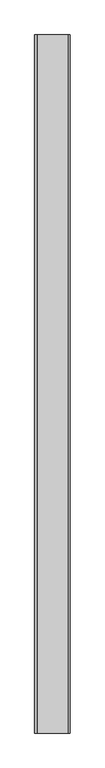
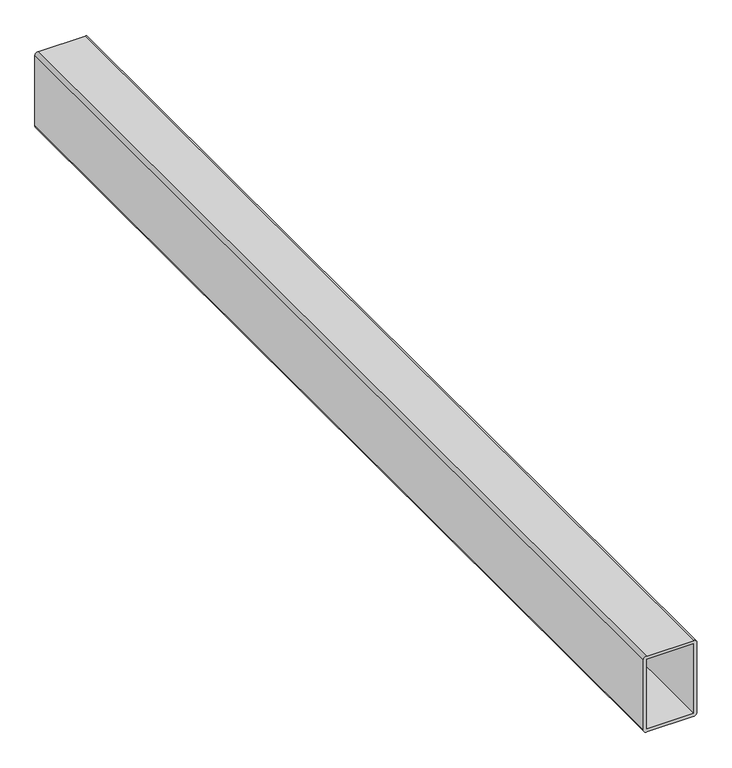
"""IFC4 building model written with IfcOpenShell, lengths in millimetres: proxy geometry, Door frame17:Door frame001:300884 : Door frame17:Door frame001:300884."""

from ifc_helpers import new_model, si_unit, point, frame, frame_2d, origin, place, context, project, spatial, polyline, circle_curve, trimmed, segment, composite_curve, outline, extrude, source, transform, mapped, element, save


def generic_models_ee08d4f9(model_context):
    return source(origin(), model_context, "Body", "SweptSolid", [
        extrude(outline(composite_curve([segment(trimmed(circle_curve(frame_2d((32622.3875625, -3620.837526)), 6.35), [point((32622.3875625, -3627.187526))], [point((32616.0375625, -3620.837526))], False, "CARTESIAN"), True, "CONTINUOUS"), segment(polyline([(32616.0375625, -3620.837526), (32616.0375625, -3531.937526)]), True, "CONTINUOUS"), segment(trimmed(circle_curve(frame_2d((32622.3875625, -3531.937526)), 6.35), [point((32616.0375625, -3531.937526))], [point((32622.3875625, -3525.587526))], False, "CARTESIAN"), True, "CONTINUOUS"), segment(polyline([(32622.3875625, -3525.587526), (32762.0875625, -3525.587526)]), True, "CONTINUOUS"), segment(trimmed(circle_curve(frame_2d((32762.0875625, -3531.937526)), 6.35), [point((32762.0875625, -3525.587526))], [point((32768.4375625, -3531.937526))], False, "CARTESIAN"), True, "CONTINUOUS"), segment(polyline([(32768.4375625, -3531.937526), (32768.4375625, -3620.837526)]), True, "CONTINUOUS"), segment(trimmed(circle_curve(frame_2d((32762.0875625, -3620.837526)), 6.35), [point((32768.4375625, -3620.837526))], [point((32762.0875625, -3627.187526))], False, "CARTESIAN"), True, "CONTINUOUS"), segment(polyline([(32762.0875625, -3627.187526), (32622.3875625, -3627.187526)]), True, "CONTINUOUS")], self_intersect=False), holes=[polyline([(32761.9375625, -3620.687526), (32761.9375625, -3532.087526), (32622.5375625, -3532.087526), (32622.5375625, -3620.687526), (32761.9375625, -3620.687526)])]), frame((0.0, 4838.7838655, 0.0), z_axis=(0.0, 1.0, 0.0), x_axis=(0.0, 0.0, 1.0)), (0.0, 0.0, 1.0), 2000.0),
    ])


if __name__ == "__main__":
    model = new_model("IFC4")
    model_context = context("Model", 3, world=origin())
    ifc_project = project(units=[si_unit("LENGTHUNIT", "METRE", prefix="MILLI")], contexts=[model_context])
    site = spatial("IfcSite", under=ifc_project)
    building = spatial("IfcBuilding", under=site)
    placement = place(None, origin())
    generic_models_shape = generic_models_ee08d4f9(model_context)
    element("IfcBuildingElementProxy", 1, Name="Door frame17:Door frame001:300884 : Door frame17:Door frame001:300884", ObjectType="Door frame17:Door frame001:300884 : Door frame17:Door frame001:300884", at=placement, inside=building, context=model_context, shape_type="MappedRepresentation", body=[
        mapped(generic_models_shape, transform((0.0, 0.0, 0.0), x_axis=(1.0, 0.0, 0.0), y_axis=(0.0, 1.0, 0.0), z_axis=(0.0, 0.0, 1.0))),
    ])
    save(model, "model.ifc")

# Revit data of these elements
# Type "Door frame17:Door frame001:300884 : Door frame17:Door frame001:300884"
#   NameOverride = "Door frame17:Door frame001:300884"
#   ObjectTypeOverride = "Door frame17:Door frame001"
#   Reference = "Door frame001"
#   Category = "Generic Models"
#   Tag = "300884"
# Element 1 (IfcBuildingElementProxy, "Door frame17:Door frame001:300884 : Door frame17:Door frame001:300884")
#   Materials on its faces: "TUBE STEEL PROFILE - METALIZED, PRIMED & PAINTED (COLOR PER ARCHITECT)"
# Materials
#   "TUBE STEEL PROFILE - METALIZED, PRIMED & PAINTED (COLOR PER ARCHITECT)": class "Unassigned", colour RGB 128 128 128, transparency 0
